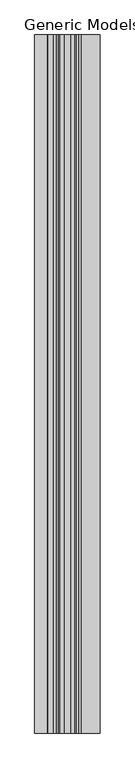
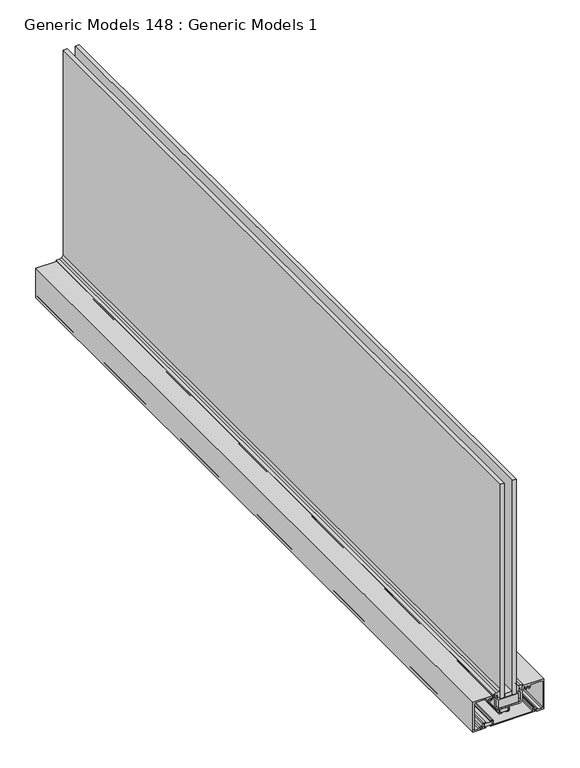
"""IFC4 building model written with IfcOpenShell, lengths in millimetres: proxy geometry, Generic Models 148 : Generic Models 1."""

import ifcopenshell
import ifcopenshell.guid

model = None  # the IFC model being written
_history = None  # IfcOwnerHistory: only IFC2X3 demands one
_inside = {}  # id of a spatial element -> (the spatial element, [elements in it])
_under = {}  # id of a project, library or spatial element -> (it, [spatial elements below it])
_declared = {}  # id of a project -> (the project, [libraries it declares])
_typed = {}  # id of a type object -> (the type object, [elements of that type])
_made_of = {}  # id of a material, layer set ... -> (it, [elements and type objects made of it])


def new_model(schema):
    """Start an empty IFC model of exactly this schema.

    Asked for "IFC4X3", IfcOpenShell would pick the latest addendum, in which some entities
    have other attributes; the version numbers below select the first issue.
    IFC2X3 requires an IfcOwnerHistory on every rooted entity: one is made here for all.
    """
    global model, _history
    if schema == "IFC4X3":
        model = ifcopenshell.file(schema_version=(4, 3, 0, 0))
    else:
        model = ifcopenshell.file(schema=schema)
    _inside.clear()
    _under.clear()
    _declared.clear()
    _typed.clear()
    _made_of.clear()
    _history = None
    if model.schema == "IFC2X3":
        org = make("IfcOrganization", Name="unknown")
        user = make(
            "IfcPersonAndOrganization",
            ThePerson=make("IfcPerson", FamilyName="unknown"),
            TheOrganization=org,
        )
        app = make(
            "IfcApplication",
            ApplicationDeveloper=org,
            Version="unknown",
            ApplicationFullName="unknown",
            ApplicationIdentifier="unknown",
        )
        _history = make(
            "IfcOwnerHistory",
            OwningUser=user,
            OwningApplication=app,
            ChangeAction="ADDED",
            CreationDate=0,
        )
    return model


def make(cls, **values):
    """One entity of the class cls with the attributes given. An attribute that is None is left unset."""
    return model.create_entity(
        cls, **{name: value for name, value in values.items() if value is not None}
    )


def rooted(cls, **values):
    """An entity with a GlobalId (a new one), such as an element, a storey or a relation."""
    return make(cls, GlobalId=ifcopenshell.guid.new(), OwnerHistory=_history, **values)


def si_unit(unit_type, name, prefix=None):
    """IfcSIUnit, for example si_unit("LENGTHUNIT", "METRE", prefix="MILLI")."""
    return make("IfcSIUnit", UnitType=unit_type, Prefix=prefix, Name=name)


def assignment(units):
    """IfcUnitAssignment: the units of a project."""
    return None if units is None else make("IfcUnitAssignment", Units=units)


def point(xyz):
    """IfcCartesianPoint."""
    return None if xyz is None else make("IfcCartesianPoint", Coordinates=xyz)


def direction(xyz):
    """IfcDirection."""
    return None if xyz is None else make("IfcDirection", DirectionRatios=xyz)


def frame(location, z_axis=None, x_axis=None):
    """IfcAxis2Placement3D, a coordinate frame: its origin and axes. An axis left out is left unset."""
    return make(
        "IfcAxis2Placement3D",
        Location=point(location),
        Axis=direction(z_axis),
        RefDirection=direction(x_axis),
    )


def frame_2d(location, x_axis=None):
    """IfcAxis2Placement2D, a coordinate frame in the plane: its origin and x axis."""
    return make(
        "IfcAxis2Placement2D", Location=point(location), RefDirection=direction(x_axis)
    )


def origin():
    """The frame at (0, 0, 0) with its axes left unset."""
    return frame((0.0, 0.0, 0.0))


def place(relative_to, where):
    """IfcLocalPlacement: puts the frame where relative to a parent placement (None: the world)."""
    return make(
        "IfcLocalPlacement", PlacementRelTo=relative_to, RelativePlacement=where
    )


def context(
    kind, dimensions, precision=None, world=None, true_north=None, identifier=None
):
    """IfcGeometricRepresentationContext, for example the 3D "Model" context."""
    return make(
        "IfcGeometricRepresentationContext",
        ContextIdentifier=identifier,
        ContextType=kind,
        CoordinateSpaceDimension=dimensions,
        Precision=precision,
        WorldCoordinateSystem=world,
        TrueNorth=true_north,
    )


def project(units=None, contexts=None):
    """IfcProject with its units and contexts."""
    return rooted(
        "IfcProject",
        Name="project",
        RepresentationContexts=contexts,
        UnitsInContext=assignment(units),
    )


def spatial(cls, under=None, at=None, **own):
    """A site, building, storey or space (cls), placed at a placement, below another one or the project."""
    s = rooted(cls, ObjectPlacement=at, **own)
    if under is not None:
        _under.setdefault(under.id(), (under, []))[1].append(s)
    return s


def polyline(points):
    """IfcPolyline through the points."""
    return make("IfcPolyline", Points=[point(p) for p in points])


def circle_curve(where, radius):
    """IfcCircle in the frame where."""
    return make("IfcCircle", Position=where, Radius=radius)


def trimmed(basis, trim1, trim2, sense, master):
    """IfcTrimmedCurve: the piece of a basis curve between two trims."""
    return make(
        "IfcTrimmedCurve",
        BasisCurve=basis,
        Trim1=trim1,
        Trim2=trim2,
        SenseAgreement=sense,
        MasterRepresentation=master,
    )


def segment(curve, same_sense, transition):
    """IfcCompositeCurveSegment."""
    return make(
        "IfcCompositeCurveSegment",
        Transition=transition,
        SameSense=same_sense,
        ParentCurve=curve,
    )


def composite_curve(segments, self_intersect=None):
    """IfcCompositeCurve: segments joined end to end."""
    return make("IfcCompositeCurve", Segments=segments, SelfIntersect=self_intersect)


def outline(outer, holes=None, kind="AREA"):
    """IfcArbitraryClosedProfileDef: a profile drawn as a closed curve; with holes, ...WithVoids."""
    if holes is None:
        return make("IfcArbitraryClosedProfileDef", ProfileType=kind, OuterCurve=outer)
    return make(
        "IfcArbitraryProfileDefWithVoids",
        ProfileType=kind,
        OuterCurve=outer,
        InnerCurves=holes,
    )


def extrude(swept, where, along, depth):
    """IfcExtrudedAreaSolid: the profile swept, set in the frame where, extruded along a direction by depth."""
    return make(
        "IfcExtrudedAreaSolid",
        SweptArea=swept,
        Position=where,
        ExtrudedDirection=direction(along),
        Depth=depth,
    )


def shape(context_of_items, identifier, shape_type, items):
    """IfcShapeRepresentation: the items that make up one representation, for example the "Body"."""
    return make(
        "IfcShapeRepresentation",
        ContextOfItems=context_of_items,
        RepresentationIdentifier=identifier,
        RepresentationType=shape_type,
        Items=items,
    )


def source(mapping_origin, context_of_items, identifier, shape_type, items):
    """IfcRepresentationMap: a shape defined once, which mapped items show again and again."""
    return make(
        "IfcRepresentationMap",
        MappingOrigin=mapping_origin,
        MappedRepresentation=shape(context_of_items, identifier, shape_type, items),
    )


def transform(
    local_origin,
    x_axis=None,
    y_axis=None,
    z_axis=None,
    scale=None,
    scale2=None,
    scale3=None,
    uniform=True,
):
    """IfcCartesianTransformationOperator3D, or its non-uniform kind. x_axis, y_axis, z_axis: its Axis1, 2, 3."""
    if uniform:
        return make(
            "IfcCartesianTransformationOperator3D",
            Axis1=direction(x_axis),
            Axis2=direction(y_axis),
            LocalOrigin=point(local_origin),
            Scale=scale,
            Axis3=direction(z_axis),
        )
    return make(
        "IfcCartesianTransformationOperator3DnonUniform",
        Axis1=direction(x_axis),
        Axis2=direction(y_axis),
        LocalOrigin=point(local_origin),
        Scale=scale,
        Axis3=direction(z_axis),
        Scale2=scale2,
        Scale3=scale3,
    )


def mapped(mapping_source, mapping_target):
    """IfcMappedItem: shows the shape of a source again, moved by a transform."""
    return make(
        "IfcMappedItem", MappingSource=mapping_source, MappingTarget=mapping_target
    )


def made_of(thing, what):
    """Note that an element or type object is made of a material, layer set ...; save() writes the relation."""
    if what is not None:
        _made_of.setdefault(what.id(), (what, []))[1].append(thing)
    return thing


def element(
    cls,
    number,
    at=None,
    inside=None,
    cuts=None,
    type_object=None,
    material=None,
    context=None,
    identifier="Body",
    shape_type=None,
    held_by="IfcProductDefinitionShape",
    body=None,
    shapes=None,
    **own,
):
    """One element of the class cls, such as IfcWall. Its Tag is "e" and its number.

    at: its placement. inside: the storey or other place that contains it. cuts: it is an
    opening in that element (IfcRelVoidsElement). A single representation is given by context,
    identifier, shape_type and body (its items); several are given by shapes. held_by: the class
    of the entity that holds the representations. save() writes the other relations.
    """
    e = rooted(cls, Tag="e%d" % number, ObjectPlacement=at, **own)
    if body is not None:
        shapes = [shape(context, identifier, shape_type, body)]
    if shapes is not None:
        e.Representation = make(held_by, Representations=shapes)
    if inside is not None:
        _inside.setdefault(inside.id(), (inside, []))[1].append(e)
    if cuts is not None:
        rooted(
            "IfcRelVoidsElement", RelatingBuildingElement=cuts, RelatedOpeningElement=e
        )
    if type_object is not None:
        _typed.setdefault(type_object.id(), (type_object, []))[1].append(e)
    return made_of(e, material)


def aggregate(whole, parts):
    """IfcRelAggregates: a whole, such as a stair, and the parts it consists of."""
    return rooted("IfcRelAggregates", RelatingObject=whole, RelatedObjects=parts)


def save(model, path):
    """Write the relations noted so far, then the file.

    IfcRelAggregates (storeys below a building ...), IfcRelContainedInSpatialStructure (elements
    in a storey), IfcRelDefinesByType, IfcRelAssociatesMaterial and IfcRelDeclares: one each for
    every whole, place, type object, material and project.
    """
    for whole, parts in _under.values():
        aggregate(whole, parts)
    for where, things in _inside.values():
        rooted(
            "IfcRelContainedInSpatialStructure",
            RelatedElements=things,
            RelatingStructure=where,
        )
    for kind, things in _typed.values():
        rooted("IfcRelDefinesByType", RelatedObjects=things, RelatingType=kind)
    for what, things in _made_of.values():
        rooted("IfcRelAssociatesMaterial", RelatedObjects=things, RelatingMaterial=what)
    for by, libraries in _declared.values():
        rooted("IfcRelDeclares", RelatingContext=by, RelatedDefinitions=libraries)
    model.write(path)


def generic_models_148_generic_models_1_015d61f0(model_context):
    return source(origin(), model_context, "Body", "SweptSolid", [
        extrude(outline(composite_curve([segment(trimmed(circle_curve(frame_2d((14.097, 50917.5916343)), 1.5795625), [point((15.6765625, 50917.5916343))], [point((14.6380548, 50916.1076271))], False, "CARTESIAN"), True, "CONTINUOUS"), segment(polyline([(14.6380548, 50916.1076271), (10.7648375, 50914.6954892), (10.7648375, 50916.1851634), (8.1835625, 50916.1851634), (8.1835625, 50911.8671634), (6.5484375, 50911.8671634), (6.5484375, 50921.1478154), (8.1835625, 50921.1478154), (8.1835625, 50917.5664154), (14.8034375, 50917.5664154), (14.8034375, 50921.1478154), (15.6765625, 50921.1478154), (15.6765625, 50917.5916343)]), True, "CONTINUOUS")], self_intersect=False)), frame((0.0, 0.0, 0.0), z_axis=(0.0, 1.0, 0.0), x_axis=(0.0, 0.0, 1.0)), (0.0, 0.0, 1.0), 1219.2),
        extrude(outline(composite_curve([segment(trimmed(circle_curve(frame_2d((12.446, 50996.7010997)), 0.7064375), [point((12.6878975, 50997.3648312))], [point((11.740864, 50996.6582372))], True, "CARTESIAN"), True, "CONTINUOUS"), segment(polyline([(11.740864, 50996.6582372), (8.1835625, 50996.6582372), (8.1835625, 50933.5636529)]), True, "CONTINUOUS"), segment(trimmed(circle_curve(frame_2d((8.89, 50933.5636529)), 0.7064375), [point((8.1835625, 50933.5636529))], [point((8.89, 50932.8572154))], True, "CARTESIAN"), True, "CONTINUOUS"), segment(polyline([(8.89, 50932.8572154), (14.097, 50932.8572154)]), True, "CONTINUOUS"), segment(trimmed(circle_curve(frame_2d((14.097, 50931.2776529)), 1.5795625), [point((14.097, 50932.8572154))], [point((15.6765625, 50931.2776529))], False, "CARTESIAN"), True, "CONTINUOUS"), segment(polyline([(15.6765625, 50931.2776529), (15.6765625, 50927.8946904), (14.8034375, 50927.8946904), (14.8034375, 50931.4760904), (8.1835625, 50931.4760904), (8.1835625, 50927.8946904), (6.5484375, 50927.8946904), (6.5484375, 51002.3573622), (8.1835625, 51002.3573622), (8.1835625, 50998.0393622), (10.7648375, 50998.0393622), (10.7648375, 50999.5290364), (16.009985, 50997.616706)]), True, "CONTINUOUS"), segment(trimmed(circle_curve(frame_2d((15.7734, 50996.9677997)), 0.6906895), [point((16.009985, 50997.616706))], [point((15.5374141, 50996.3186752))], False, "CARTESIAN"), True, "CONTINUOUS"), segment(polyline([(15.5374141, 50996.3186752), (12.6878975, 50997.3648312)]), True, "CONTINUOUS")], self_intersect=False)), frame((0.0, 0.0, 0.0), z_axis=(0.0, 1.0, 0.0), x_axis=(0.0, 0.0, 1.0)), (0.0, 0.0, 1.0), 1219.2),
        extrude(outline(composite_curve([segment(trimmed(circle_curve(frame_2d((34.29, 50974.625)), 2.54), [point((34.29, 50977.165))], [point((31.75, 50974.625))], True, "CARTESIAN"), True, "CONTINUOUS"), segment(polyline([(31.75, 50974.625), (31.75, 50953.1493), (29.718, 50953.1493), (29.718, 50956.7307), (23.495, 50956.7307), (23.495, 50953.1493), (22.225, 50953.1493), (22.225, 50956.7307)]), True, "CONTINUOUS"), segment(trimmed(circle_curve(frame_2d((24.003, 50956.7307)), 1.778), [point((22.225, 50956.7307))], [point((24.003, 50958.5087))], False, "CARTESIAN"), True, "CONTINUOUS"), segment(polyline([(24.003, 50958.5087), (29.21, 50958.5087)]), True, "CONTINUOUS"), segment(trimmed(circle_curve(frame_2d((29.21, 50959.0167)), 0.508), [point((29.21, 50958.5087))], [point((29.718, 50959.0167))], True, "CARTESIAN"), True, "CONTINUOUS"), segment(polyline([(29.718, 50959.0167), (29.718, 50974.879)]), True, "CONTINUOUS"), segment(trimmed(circle_curve(frame_2d((34.036, 50974.879)), 4.318), [point((29.718, 50974.879))], [point((34.036, 50979.197))], False, "CARTESIAN"), True, "CONTINUOUS"), segment(polyline([(34.036, 50979.197), (49.1342256, 50979.197), (50.8386835, 50980.9028737)]), True, "CONTINUOUS"), segment(trimmed(circle_curve(frame_2d((52.7253201, 50979.017803)), 2.667), [point((50.8386835, 50980.9028737))], [point((52.7253201, 50981.684803))], False, "CARTESIAN"), True, "CONTINUOUS"), segment(polyline([(52.7253201, 50981.684803), (54.61, 50981.684803)]), True, "CONTINUOUS"), segment(trimmed(circle_curve(frame_2d((54.61, 50982.192803)), 0.508), [point((54.61, 50981.684803))], [point((55.118, 50982.192803))], True, "CARTESIAN"), True, "CONTINUOUS"), segment(polyline([(55.118, 50982.192803), (55.118, 50984.0043351)]), True, "CONTINUOUS"), segment(trimmed(circle_curve(frame_2d((54.61, 50984.0043351)), 0.508), [point((55.118, 50984.0043351))], [point((54.3683568, 50984.4511825))], True, "CARTESIAN"), True, "CONTINUOUS"), segment(trimmed(circle_curve(frame_2d((52.3748, 50988.137673)), 4.191), [point((54.3683568, 50984.4511825))], [point((49.3268, 50985.2611861))], False, "CARTESIAN"), True, "CONTINUOUS"), segment(polyline([(49.3268, 50985.2611861), (49.3268, 50986.3779094), (50.2850807, 50986.931173)]), True, "CONTINUOUS"), segment(trimmed(circle_curve(frame_2d((52.3748, 50988.137673)), 2.413), [point((50.2850807, 50986.931173))], [point((50.2850807, 50989.344173))], True, "CARTESIAN"), True, "CONTINUOUS"), segment(polyline([(50.2850807, 50989.344173), (49.3268, 50989.8974366), (49.3268, 50991.0141599)]), True, "CONTINUOUS"), segment(trimmed(circle_curve(frame_2d((52.3748, 50988.137673)), 4.191), [point((49.3268, 50991.0141599))], [point((54.3683568, 50991.8241635))], False, "CARTESIAN"), True, "CONTINUOUS"), segment(trimmed(circle_curve(frame_2d((54.61, 50992.2710109)), 0.508), [point((54.3683568, 50991.8241635))], [point((55.118, 50992.2710109))], True, "CARTESIAN"), True, "CONTINUOUS"), segment(polyline([(55.118, 50992.2710109), (55.118, 51010.756373)]), True, "CONTINUOUS"), segment(trimmed(circle_curve(frame_2d((53.594, 51010.756373)), 1.524), [point((55.118, 51010.756373))], [point((53.594, 51012.280373))], True, "CARTESIAN"), True, "CONTINUOUS"), segment(polyline([(53.594, 51012.280373), (9.906, 51012.280373)]), True, "CONTINUOUS"), segment(trimmed(circle_curve(frame_2d((9.906, 51010.756373)), 1.524), [point((9.906, 51012.280373))], [point((8.382, 51010.756373))], True, "CARTESIAN"), True, "CONTINUOUS"), segment(polyline([(8.382, 51010.756373), (8.382, 51004.700214)]), True, "CONTINUOUS"), segment(trimmed(circle_curve(frame_2d((8.89, 51003.263373)), 1.524), [point((8.382, 51004.700214))], [point((10.414, 51003.263373))], False, "CARTESIAN"), True, "CONTINUOUS"), segment(polyline([(10.414, 51003.263373), (10.414, 50998.5052015)]), True, "CONTINUOUS"), segment(trimmed(circle_curve(frame_2d((9.9568, 51000.012173)), 1.5748), [point((10.414, 50998.5052015))], [point((8.382, 51000.012173))], False, "CARTESIAN"), True, "CONTINUOUS"), segment(polyline([(8.382, 51000.012173), (8.382, 51002.755373), (6.35, 51002.755373), (6.35, 51014.312373), (57.15, 51014.312373), (57.15, 50979.652803), (52.46214, 50979.652803), (50.5841, 50977.773203), (50.5841, 50976.2991491), (53.5813, 50975.640873), (55.3593, 50975.640873), (55.3593, 50974.624873), (49.3141, 50974.624873), (49.3141, 50976.657)]), True, "CONTINUOUS"), segment(trimmed(circle_curve(frame_2d((48.8061, 50976.657)), 0.508), [point((49.3141, 50976.657))], [point((48.8061, 50977.165))], True, "CARTESIAN"), True, "CONTINUOUS"), segment(polyline([(48.8061, 50977.165), (34.29, 50977.165)]), True, "CONTINUOUS")], self_intersect=False)), frame((0.0, 0.0, 0.0), z_axis=(0.0, 1.0, 0.0), x_axis=(0.0, 0.0, 1.0)), (0.0, 0.0, 1.0), 1219.2),
        extrude(outline(composite_curve([segment(trimmed(circle_curve(frame_2d((48.8061, 50937.667873)), 0.508), [point((48.8061, 50937.159873))], [point((49.3141, 50937.667873))], True, "CARTESIAN"), True, "CONTINUOUS"), segment(polyline([(49.3141, 50937.667873), (49.3141, 50939.7), (55.3593, 50939.7), (55.3593, 50938.684), (53.5813, 50938.684), (50.5841, 50938.0257239), (50.5841, 50936.55167), (52.46214, 50934.67207), (57.15, 50934.67207), (57.15, 50900.0125), (6.35, 50900.0125), (6.35, 50911.5695), (8.382, 50911.5695), (8.382, 50914.3127)]), True, "CONTINUOUS"), segment(trimmed(circle_curve(frame_2d((9.9568, 50914.3127)), 1.5748), [point((8.382, 50914.3127))], [point((10.414, 50915.8196715))], False, "CARTESIAN"), True, "CONTINUOUS"), segment(polyline([(10.414, 50915.8196715), (10.414, 50911.0615)]), True, "CONTINUOUS"), segment(trimmed(circle_curve(frame_2d((8.89, 50911.0615)), 1.524), [point((10.414, 50911.0615))], [point((8.382, 50909.624659))], False, "CARTESIAN"), True, "CONTINUOUS"), segment(polyline([(8.382, 50909.624659), (8.382, 50903.568373)]), True, "CONTINUOUS"), segment(trimmed(circle_curve(frame_2d((9.906, 50903.568373)), 1.524), [point((8.382, 50903.568373))], [point((9.906, 50902.044373))], True, "CARTESIAN"), True, "CONTINUOUS"), segment(polyline([(9.906, 50902.044373), (53.594, 50902.044373)]), True, "CONTINUOUS"), segment(trimmed(circle_curve(frame_2d((53.594, 50903.568373)), 1.524), [point((53.594, 50902.044373))], [point((55.118, 50903.568373))], True, "CARTESIAN"), True, "CONTINUOUS"), segment(polyline([(55.118, 50903.568373), (55.118, 50922.0538621)]), True, "CONTINUOUS"), segment(trimmed(circle_curve(frame_2d((54.61, 50922.0538621)), 0.508), [point((55.118, 50922.0538621))], [point((54.3683568, 50922.5007095))], True, "CARTESIAN"), True, "CONTINUOUS"), segment(trimmed(circle_curve(frame_2d((52.3748, 50926.1872)), 4.191), [point((54.3683568, 50922.5007095))], [point((49.3268, 50923.3107131))], False, "CARTESIAN"), True, "CONTINUOUS"), segment(polyline([(49.3268, 50923.3107131), (49.3268, 50924.4274364), (50.2850807, 50924.9807)]), True, "CONTINUOUS"), segment(trimmed(circle_curve(frame_2d((52.3748, 50926.1872)), 2.413), [point((50.2850807, 50924.9807))], [point((50.2850807, 50927.3937))], True, "CARTESIAN"), True, "CONTINUOUS"), segment(polyline([(50.2850807, 50927.3937), (49.3268, 50927.9469636), (49.3268, 50929.0636869)]), True, "CONTINUOUS"), segment(trimmed(circle_curve(frame_2d((52.3748, 50926.1872)), 4.191), [point((49.3268, 50929.0636869))], [point((54.3683568, 50929.8736905))], False, "CARTESIAN"), True, "CONTINUOUS"), segment(trimmed(circle_curve(frame_2d((54.61, 50930.3205379)), 0.508), [point((54.3683568, 50929.8736905))], [point((55.118, 50930.3205379))], True, "CARTESIAN"), True, "CONTINUOUS"), segment(polyline([(55.118, 50930.3205379), (55.118, 50932.13207)]), True, "CONTINUOUS"), segment(trimmed(circle_curve(frame_2d((54.61, 50932.13207)), 0.508), [point((55.118, 50932.13207))], [point((54.61, 50932.64007))], True, "CARTESIAN"), True, "CONTINUOUS"), segment(polyline([(54.61, 50932.64007), (52.7253201, 50932.64007)]), True, "CONTINUOUS"), segment(trimmed(circle_curve(frame_2d((52.7253201, 50935.30707)), 2.667), [point((52.7253201, 50932.64007))], [point((50.8386835, 50933.4219993))], False, "CARTESIAN"), True, "CONTINUOUS"), segment(polyline([(50.8386835, 50933.4219993), (49.1342256, 50935.127873), (34.036, 50935.127873)]), True, "CONTINUOUS"), segment(trimmed(circle_curve(frame_2d((34.036, 50939.445873)), 4.318), [point((34.036, 50935.127873))], [point((29.718, 50939.445873))], False, "CARTESIAN"), True, "CONTINUOUS"), segment(polyline([(29.718, 50939.445873), (29.718, 50941.439773), (24.003, 50941.439773)]), True, "CONTINUOUS"), segment(trimmed(circle_curve(frame_2d((24.003, 50943.217773)), 1.778), [point((24.003, 50941.439773))], [point((22.225, 50943.217773))], False, "CARTESIAN"), True, "CONTINUOUS"), segment(polyline([(22.225, 50943.217773), (22.225, 50946.7993), (23.495, 50946.7993), (23.495, 50943.2179), (29.718, 50943.2179), (29.718, 50946.7993), (31.75, 50946.7993), (31.75, 50939.699873)]), True, "CONTINUOUS"), segment(trimmed(circle_curve(frame_2d((34.29, 50939.699873)), 2.54), [point((31.75, 50939.699873))], [point((34.29, 50937.159873))], True, "CARTESIAN"), True, "CONTINUOUS"), segment(polyline([(34.29, 50937.159873), (48.8061, 50937.159873)]), True, "CONTINUOUS")], self_intersect=False)), frame((0.0, 0.0, 0.0), z_axis=(0.0, 1.0, 0.0), x_axis=(0.0, 0.0, 1.0)), (0.0, 0.0, 1.0), 1219.2),
        extrude(outline(polyline([(50973.0629678, 0.0), (50941.7098428, 0.0), (50941.7098428, 1219.2), (50973.0629678, 1219.2), (50973.0629678, 0.0)])), frame((0.0, 0.0, 32.5992301), z_axis=(0.0, 0.0, 1.0), x_axis=(1.0, 0.0, 0.0)), (0.0, 0.0, 1.0), 14.684375),
        extrude(outline(polyline([(50950.82359, 0.0), (50944.47359, 0.0), (50944.47359, 1219.2), (50950.82359, 1219.2), (50950.82359, 0.0)])), frame((0.0, 0.0, 47.625), z_axis=(0.0, 0.0, 1.0), x_axis=(1.0, 0.0, 0.0)), (0.0, 0.0, 1.0), 365.125),
        extrude(outline(polyline([(50969.87359, 0.0), (50963.52359, 0.0), (50963.52359, 1219.2), (50969.87359, 1219.2), (50969.87359, 0.0)])), frame((0.0, 0.0, 47.625), z_axis=(0.0, 0.0, 1.0), x_axis=(1.0, 0.0, 0.0)), (0.0, 0.0, 1.0), 365.125),
        extrude(outline(polyline([(50963.3251525, 0.0), (50951.0220275, 0.0), (50951.0220275, 1219.2), (50963.3251525, 1219.2), (50963.3251525, 0.0)])), frame((0.0, 0.0, 47.625), z_axis=(0.0, 0.0, 1.0), x_axis=(1.0, 0.0, 0.0)), (0.0, 0.0, 1.0), 6.35),
        extrude(outline(composite_curve([segment(trimmed(circle_curve(frame_2d((64.2304882, 50976.1426745)), 4.9643345), [point((59.3077698, 50976.7841265))], [point((60.6315489, 50972.7232808))], True, "CARTESIAN"), True, "CONTINUOUS"), segment(polyline([(60.6315489, 50972.7232808), (63.5908154, 50970.1744071), (50.679329, 50970.1744071), (50.679329, 50974.1558571), (56.1304866, 50974.1558571), (56.1304866, 50975.8945302), (54.2354153, 50975.8945302), (51.2348926, 50976.553536), (51.2348926, 50977.5441268), (52.8805452, 50979.1911463), (57.5342084, 50979.1911463), (57.5342084, 50980.9684916), (58.6865882, 50980.9684916)]), True, "CONTINUOUS"), segment(trimmed(circle_curve(frame_2d((47.3152777, 50977.1420956)), 11.9978335), [point((58.6865882, 50980.9684916))], [point((59.3077698, 50976.7841265))], False, "CARTESIAN"), True, "CONTINUOUS")], self_intersect=False)), frame((0.0, 0.0, 0.0), z_axis=(0.0, 1.0, 0.0), x_axis=(0.0, 0.0, 1.0)), (0.0, 0.0, 1.0), 1219.2),
        extrude(outline(composite_curve([segment(trimmed(circle_curve(frame_2d((47.3152777, 50937.0578364)), 11.9978335), [point((59.3077698, 50937.4158055))], [point((58.6865882, 50933.2314404))], False, "CARTESIAN"), True, "CONTINUOUS"), segment(polyline([(58.6865882, 50933.2314404), (57.5342084, 50933.2314404), (57.5342084, 50935.0087857), (52.8805452, 50935.0087857), (51.2348926, 50936.6558052), (51.2348926, 50937.646396), (54.2354153, 50938.3054018), (56.1304866, 50938.3054018), (56.1304866, 50940.0440749), (50.679329, 50940.0440749), (50.679329, 50944.0255249), (63.5908154, 50944.0255249), (60.6315489, 50941.4766512)]), True, "CONTINUOUS"), segment(trimmed(circle_curve(frame_2d((64.2304882, 50938.0572575)), 4.9643345), [point((60.6315489, 50941.4766512))], [point((59.3077698, 50937.4158055))], True, "CARTESIAN"), True, "CONTINUOUS")], self_intersect=False)), frame((0.0, 0.0, 0.0), z_axis=(0.0, 1.0, 0.0), x_axis=(0.0, 0.0, 1.0)), (0.0, 0.0, 1.0), 1219.2),
        extrude(outline(polyline([(50931.0792154, 0.0), (50917.9632904, 0.0), (50917.9632904, 1219.2), (50931.0792154, 1219.2), (50931.0792154, 0.0)])), frame((0.0, 0.0, 8.5804375), z_axis=(0.0, 0.0, 1.0), x_axis=(1.0, 0.0, 0.0)), (0.0, 0.0, 1.0), 5.826125),
        extrude(outline(polyline([(50956.5322625, 0.0), (50943.4163375, 0.0), (50943.4163375, 1219.2), (50956.5322625, 1219.2), (50956.5322625, 0.0)])), frame((0.0, 0.0, 23.6934375), z_axis=(0.0, 0.0, 1.0), x_axis=(1.0, 0.0, 0.0)), (0.0, 0.0, 1.0), 5.826125),
    ])


if __name__ == "__main__":
    model = new_model("IFC4")
    model_context = context("Model", 3, world=origin())
    ifc_project = project(units=[si_unit("LENGTHUNIT", "METRE", prefix="MILLI")], contexts=[model_context])
    site = spatial("IfcSite", under=ifc_project)
    building = spatial("IfcBuilding", under=site)
    placement = place(None, origin())
    generic_models_148_generic_models_1_shape = generic_models_148_generic_models_1_015d61f0(model_context)
    element("IfcBuildingElementProxy", 1, Name="Generic Models 148 : Generic Models 1", ObjectType="Generic Models 148 : Generic Models 1", at=placement, inside=building, context=model_context, shape_type="MappedRepresentation", body=[
        mapped(generic_models_148_generic_models_1_shape, transform((0.0, 0.0, 0.0), x_axis=(1.0, 0.0, 0.0), y_axis=(0.0, 1.0, 0.0), z_axis=(0.0, 0.0, 1.0))),
    ])
    save(model, "model.ifc")

# Revit data of these elements
# Element 1 (IfcBuildingElementProxy, "Generic Models 148 : Generic Models 1")
#   Materials on its faces: "ALUM. STOREFRONT W/ INSULATED GLAZING"
# Materials
#   "ALUM. STOREFRONT W/ INSULATED GLAZING": class "Glass", colour RGB 196 205 210, transparency 0.85, Description = "Soda Lime Glass", Cost = 0
